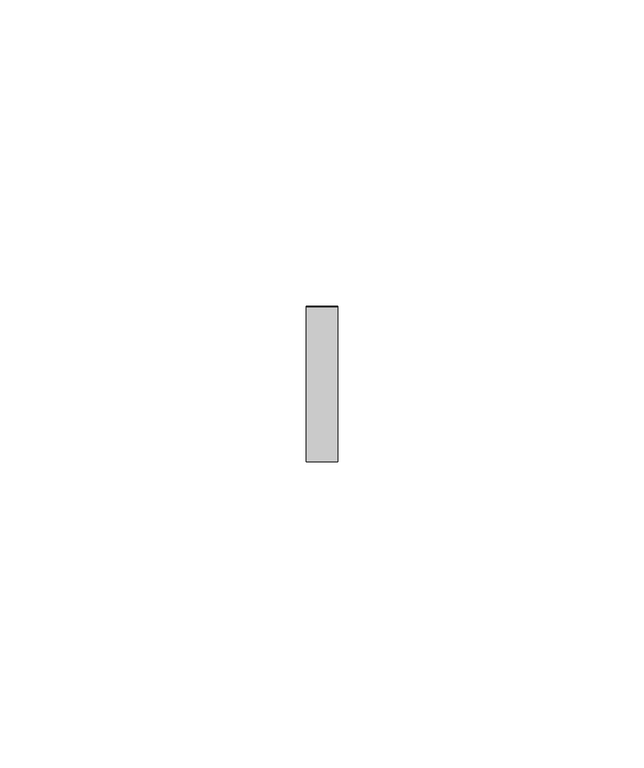
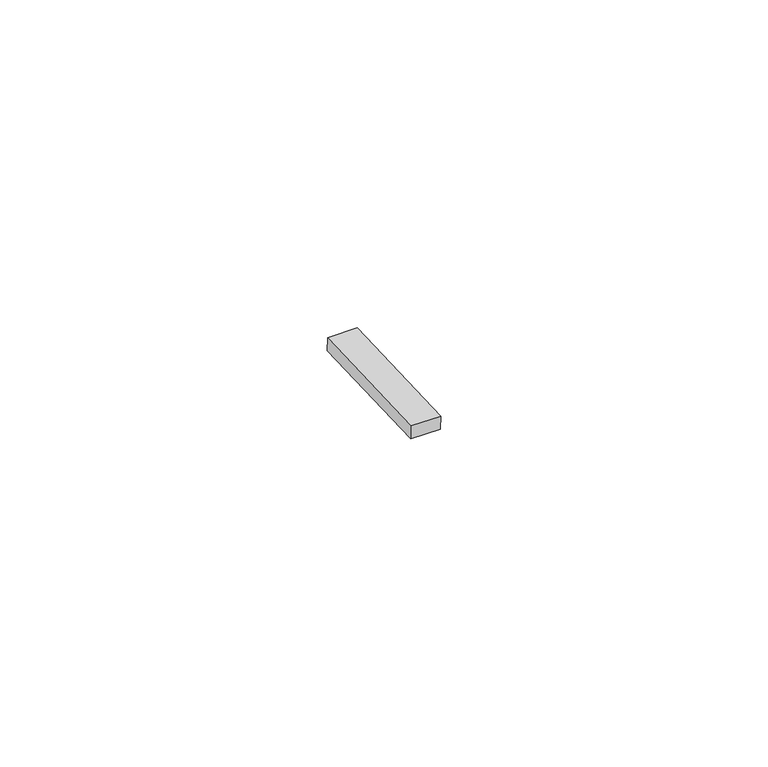
"""IFC4 building model written with IfcOpenShell, lengths in millimetres: proxy geometry, Inner panel:Inner panel:1:Inner panel:1 : Inner panel:Inner panel:300324:2:Inner panel:1:Inner panel:1 : Inner panel:Inner panel:300324:2 : Inner panel:Inner panel:1:Inner panel:1 : Inner panel:Inner panel:300324:300043:123 : Inner panel:Inner panel:1:Inner panel:1 : Inner panel:Inner panel:300324:2:Inner panel:1:Inner panel:1 : Inner panel:Inner panel:300324:2 : Inner panel:Inner panel:1:Inner panel:1 : Inner panel:Inner panel:300324:300043:308120."""

import ifcopenshell
import ifcopenshell.guid

model = None  # the IFC model being written
_history = None  # IfcOwnerHistory: only IFC2X3 demands one
_inside = {}  # id of a spatial element -> (the spatial element, [elements in it])
_under = {}  # id of a project, library or spatial element -> (it, [spatial elements below it])
_declared = {}  # id of a project -> (the project, [libraries it declares])
_typed = {}  # id of a type object -> (the type object, [elements of that type])
_made_of = {}  # id of a material, layer set ... -> (it, [elements and type objects made of it])


def new_model(schema):
    """Start an empty IFC model of exactly this schema.

    Asked for "IFC4X3", IfcOpenShell would pick the latest addendum, in which some entities
    have other attributes; the version numbers below select the first issue.
    IFC2X3 requires an IfcOwnerHistory on every rooted entity: one is made here for all.
    """
    global model, _history
    if schema == "IFC4X3":
        model = ifcopenshell.file(schema_version=(4, 3, 0, 0))
    else:
        model = ifcopenshell.file(schema=schema)
    _inside.clear()
    _under.clear()
    _declared.clear()
    _typed.clear()
    _made_of.clear()
    _history = None
    if model.schema == "IFC2X3":
        org = make("IfcOrganization", Name="unknown")
        user = make(
            "IfcPersonAndOrganization",
            ThePerson=make("IfcPerson", FamilyName="unknown"),
            TheOrganization=org,
        )
        app = make(
            "IfcApplication",
            ApplicationDeveloper=org,
            Version="unknown",
            ApplicationFullName="unknown",
            ApplicationIdentifier="unknown",
        )
        _history = make(
            "IfcOwnerHistory",
            OwningUser=user,
            OwningApplication=app,
            ChangeAction="ADDED",
            CreationDate=0,
        )
    return model


def make(cls, **values):
    """One entity of the class cls with the attributes given. An attribute that is None is left unset."""
    return model.create_entity(
        cls, **{name: value for name, value in values.items() if value is not None}
    )


def rooted(cls, **values):
    """An entity with a GlobalId (a new one), such as an element, a storey or a relation."""
    return make(cls, GlobalId=ifcopenshell.guid.new(), OwnerHistory=_history, **values)


def si_unit(unit_type, name, prefix=None):
    """IfcSIUnit, for example si_unit("LENGTHUNIT", "METRE", prefix="MILLI")."""
    return make("IfcSIUnit", UnitType=unit_type, Prefix=prefix, Name=name)


def assignment(units):
    """IfcUnitAssignment: the units of a project."""
    return None if units is None else make("IfcUnitAssignment", Units=units)


def point(xyz):
    """IfcCartesianPoint."""
    return None if xyz is None else make("IfcCartesianPoint", Coordinates=xyz)


def direction(xyz):
    """IfcDirection."""
    return None if xyz is None else make("IfcDirection", DirectionRatios=xyz)


def frame(location, z_axis=None, x_axis=None):
    """IfcAxis2Placement3D, a coordinate frame: its origin and axes. An axis left out is left unset."""
    return make(
        "IfcAxis2Placement3D",
        Location=point(location),
        Axis=direction(z_axis),
        RefDirection=direction(x_axis),
    )


def origin():
    """The frame at (0, 0, 0) with its axes left unset."""
    return frame((0.0, 0.0, 0.0))


def place(relative_to, where):
    """IfcLocalPlacement: puts the frame where relative to a parent placement (None: the world)."""
    return make(
        "IfcLocalPlacement", PlacementRelTo=relative_to, RelativePlacement=where
    )


def context(
    kind, dimensions, precision=None, world=None, true_north=None, identifier=None
):
    """IfcGeometricRepresentationContext, for example the 3D "Model" context."""
    return make(
        "IfcGeometricRepresentationContext",
        ContextIdentifier=identifier,
        ContextType=kind,
        CoordinateSpaceDimension=dimensions,
        Precision=precision,
        WorldCoordinateSystem=world,
        TrueNorth=true_north,
    )


def project(units=None, contexts=None):
    """IfcProject with its units and contexts."""
    return rooted(
        "IfcProject",
        Name="project",
        RepresentationContexts=contexts,
        UnitsInContext=assignment(units),
    )


def spatial(cls, under=None, at=None, **own):
    """A site, building, storey or space (cls), placed at a placement, below another one or the project."""
    s = rooted(cls, ObjectPlacement=at, **own)
    if under is not None:
        _under.setdefault(under.id(), (under, []))[1].append(s)
    return s


def polyline(points):
    """IfcPolyline through the points."""
    return make("IfcPolyline", Points=[point(p) for p in points])


def outline(outer, holes=None, kind="AREA"):
    """IfcArbitraryClosedProfileDef: a profile drawn as a closed curve; with holes, ...WithVoids."""
    if holes is None:
        return make("IfcArbitraryClosedProfileDef", ProfileType=kind, OuterCurve=outer)
    return make(
        "IfcArbitraryProfileDefWithVoids",
        ProfileType=kind,
        OuterCurve=outer,
        InnerCurves=holes,
    )


def extrude(swept, where, along, depth):
    """IfcExtrudedAreaSolid: the profile swept, set in the frame where, extruded along a direction by depth."""
    return make(
        "IfcExtrudedAreaSolid",
        SweptArea=swept,
        Position=where,
        ExtrudedDirection=direction(along),
        Depth=depth,
    )


def shape(context_of_items, identifier, shape_type, items):
    """IfcShapeRepresentation: the items that make up one representation, for example the "Body"."""
    return make(
        "IfcShapeRepresentation",
        ContextOfItems=context_of_items,
        RepresentationIdentifier=identifier,
        RepresentationType=shape_type,
        Items=items,
    )


def source(mapping_origin, context_of_items, identifier, shape_type, items):
    """IfcRepresentationMap: a shape defined once, which mapped items show again and again."""
    return make(
        "IfcRepresentationMap",
        MappingOrigin=mapping_origin,
        MappedRepresentation=shape(context_of_items, identifier, shape_type, items),
    )


def transform(
    local_origin,
    x_axis=None,
    y_axis=None,
    z_axis=None,
    scale=None,
    scale2=None,
    scale3=None,
    uniform=True,
):
    """IfcCartesianTransformationOperator3D, or its non-uniform kind. x_axis, y_axis, z_axis: its Axis1, 2, 3."""
    if uniform:
        return make(
            "IfcCartesianTransformationOperator3D",
            Axis1=direction(x_axis),
            Axis2=direction(y_axis),
            LocalOrigin=point(local_origin),
            Scale=scale,
            Axis3=direction(z_axis),
        )
    return make(
        "IfcCartesianTransformationOperator3DnonUniform",
        Axis1=direction(x_axis),
        Axis2=direction(y_axis),
        LocalOrigin=point(local_origin),
        Scale=scale,
        Axis3=direction(z_axis),
        Scale2=scale2,
        Scale3=scale3,
    )


def mapped(mapping_source, mapping_target):
    """IfcMappedItem: shows the shape of a source again, moved by a transform."""
    return make(
        "IfcMappedItem", MappingSource=mapping_source, MappingTarget=mapping_target
    )


def made_of(thing, what):
    """Note that an element or type object is made of a material, layer set ...; save() writes the relation."""
    if what is not None:
        _made_of.setdefault(what.id(), (what, []))[1].append(thing)
    return thing


def element(
    cls,
    number,
    at=None,
    inside=None,
    cuts=None,
    type_object=None,
    material=None,
    context=None,
    identifier="Body",
    shape_type=None,
    held_by="IfcProductDefinitionShape",
    body=None,
    shapes=None,
    **own,
):
    """One element of the class cls, such as IfcWall. Its Tag is "e" and its number.

    at: its placement. inside: the storey or other place that contains it. cuts: it is an
    opening in that element (IfcRelVoidsElement). A single representation is given by context,
    identifier, shape_type and body (its items); several are given by shapes. held_by: the class
    of the entity that holds the representations. save() writes the other relations.
    """
    e = rooted(cls, Tag="e%d" % number, ObjectPlacement=at, **own)
    if body is not None:
        shapes = [shape(context, identifier, shape_type, body)]
    if shapes is not None:
        e.Representation = make(held_by, Representations=shapes)
    if inside is not None:
        _inside.setdefault(inside.id(), (inside, []))[1].append(e)
    if cuts is not None:
        rooted(
            "IfcRelVoidsElement", RelatingBuildingElement=cuts, RelatedOpeningElement=e
        )
    if type_object is not None:
        _typed.setdefault(type_object.id(), (type_object, []))[1].append(e)
    return made_of(e, material)


def aggregate(whole, parts):
    """IfcRelAggregates: a whole, such as a stair, and the parts it consists of."""
    return rooted("IfcRelAggregates", RelatingObject=whole, RelatedObjects=parts)


def save(model, path):
    """Write the relations noted so far, then the file.

    IfcRelAggregates (storeys below a building ...), IfcRelContainedInSpatialStructure (elements
    in a storey), IfcRelDefinesByType, IfcRelAssociatesMaterial and IfcRelDeclares: one each for
    every whole, place, type object, material and project.
    """
    for whole, parts in _under.values():
        aggregate(whole, parts)
    for where, things in _inside.values():
        rooted(
            "IfcRelContainedInSpatialStructure",
            RelatedElements=things,
            RelatingStructure=where,
        )
    for kind, things in _typed.values():
        rooted("IfcRelDefinesByType", RelatedObjects=things, RelatingType=kind)
    for what, things in _made_of.values():
        rooted("IfcRelAssociatesMaterial", RelatedObjects=things, RelatingMaterial=what)
    for by, libraries in _declared.values():
        rooted("IfcRelDeclares", RelatingContext=by, RelatedDefinitions=libraries)
    model.write(path)


def generic_models_119eee7f(model_context):
    return source(origin(), model_context, "Body", "SweptSolid", [
        extrude(outline(polyline([(0.0, -25.4), (0.0, 0.0), (5.2138089, 0.0), (5.2138089, -25.4), (0.0, -25.4)])), frame((592717.395117, -578253.2828061, 3981.0403755), z_axis=(0.0, -0.041630544712223896, 0.9991330730923502), x_axis=(-1.0, 0.0, 0.0)), (0.0, 0.0, 1.0), 2.4763745),
    ])


if __name__ == "__main__":
    model = new_model("IFC4")
    model_context = context("Model", 3, world=origin())
    ifc_project = project(units=[si_unit("LENGTHUNIT", "METRE", prefix="MILLI")], contexts=[model_context])
    site = spatial("IfcSite", under=ifc_project)
    building = spatial("IfcBuilding", under=site)
    placement = place(None, origin())
    generic_models_shape = generic_models_119eee7f(model_context)
    element("IfcBuildingElementProxy", 1, Name="Inner panel:Inner panel:1:Inner panel:1 : Inner panel:Inner panel:300324:2:Inner panel:1:Inner panel:1 : Inner panel:Inner panel:300324:2 : Inner panel:Inner panel:1:Inner panel:1 : Inner panel:Inner panel:300324:300043:123 : Inner panel:Inner panel:1:Inner panel:1 : Inner panel:Inner panel:300324:2:Inner panel:1:Inner panel:1 : Inner panel:Inner panel:300324:2 : Inner panel:Inner panel:1:Inner panel:1 : Inner panel:Inner panel:300324:300043:308120", ObjectType="Inner panel:Inner panel:1:Inner panel:1 : Inner panel:Inner panel:300324:2:Inner panel:1:Inner panel:1 : Inner panel:Inner panel:300324:2 : Inner panel:Inner panel:1:Inner panel:1 : Inner panel:Inner panel:300324:300043:123 : Inner panel:Inner panel:1:Inner panel:1 : Inner panel:Inner panel:300324:2:Inner panel:1:Inner panel:1 : Inner panel:Inner panel:300324:2 : Inner panel:Inner panel:1:Inner panel:1 : Inner panel:Inner panel:300324:300043:308120", at=placement, inside=building, context=model_context, shape_type="MappedRepresentation", body=[
        mapped(generic_models_shape, transform((0.0, 0.0, 0.0), x_axis=(1.0, 0.0, 0.0), y_axis=(0.0, 1.0, 0.0), z_axis=(0.0, 0.0, 1.0))),
    ])
    save(model, "model.ifc")

# Revit data of these elements
# Type "Inner panel:Inner panel:1:Inner panel:1 : Inner panel:Inner panel:300324:2:Inner panel:1:Inner panel:1 : Inner panel:Inner panel:300324:2 : Inner panel:Inner panel:1:Inner panel:1 : Inner panel:Inner panel:300324:300043:123 : Inner panel:Inner panel:1:Inner panel:1 : Inner panel:Inner panel:300324:2:Inner panel:1:Inner panel:1 : Inner panel:Inner panel:300324:2 : Inner panel:Inner panel:1:Inner panel:1 : Inner panel:Inner panel:300324:300043:308120"
#   NameOverride = "Inner panel:Inner panel:1:Inner panel:1 : Inner panel:Inner panel:300324:2:Inner panel:1:Inner panel:1 : Inner panel:Inner panel:300324:2 : Inner panel:Inner panel:1:Inner panel:1 : Inner panel:Inner panel:300324:300043:308120"
#   ObjectTypeOverride = "Inner panel:1:Inner panel:1 : Inner panel:Inner panel:300324:2 : Inner panel:Inner panel:1:Inner panel:1 : Inner panel:Inner panel:300324:300043"
#   Reference = "Inner panel"
#   Tag = "308120"
# Element 1 (IfcBuildingElementProxy, "Inner panel:Inner panel:1:Inner panel:1 : Inner panel:Inner panel:300324:2:Inner panel:1:Inner panel:1 : Inner panel:Inner panel:300324:2 : Inner panel:Inner panel:1:Inner panel:1 : Inner panel:Inner panel:300324:300043:123 : Inner panel:Inner panel:1:Inner panel:1 : Inner panel:Inner panel:300324:2:Inner panel:1:Inner panel:1 : Inner panel:Inner panel:300324:2 : Inner panel:Inner panel:1:Inner panel:1 : Inner panel:Inner panel:300324:300043:308120")
#   Materials on its faces: "AT CLIP - 1\" WIDE NON ABSORBENT, WEATHER-RESISTANT NEOPRENE/EPDM/SBR FOAM"
# Materials
#   "AT CLIP - 1\" WIDE NON ABSORBENT, WEATHER-RESISTANT NEOPRENE/EPDM/SBR FOAM": class "Generic", colour RGB 85 85 85, transparency 0, Cost = 0
